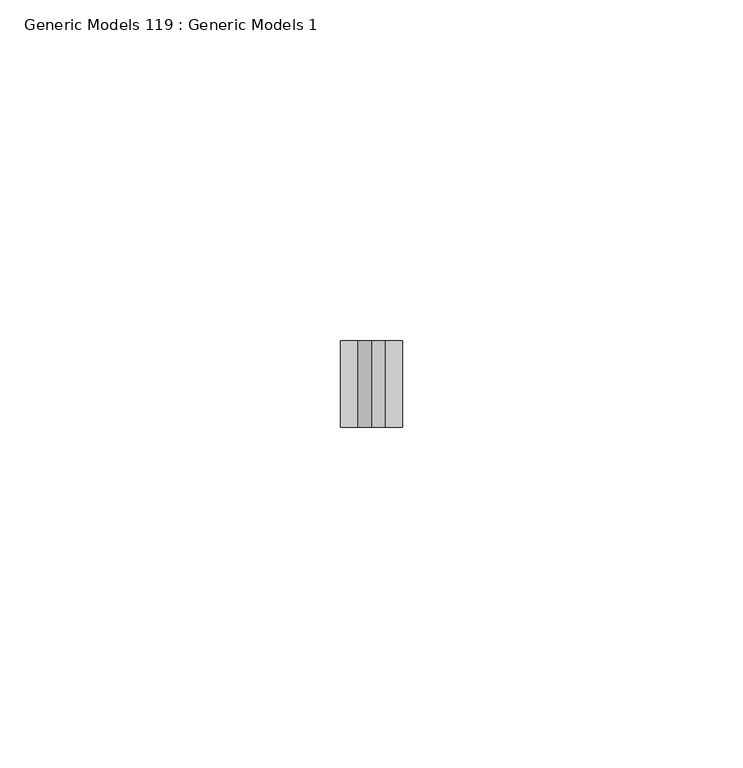
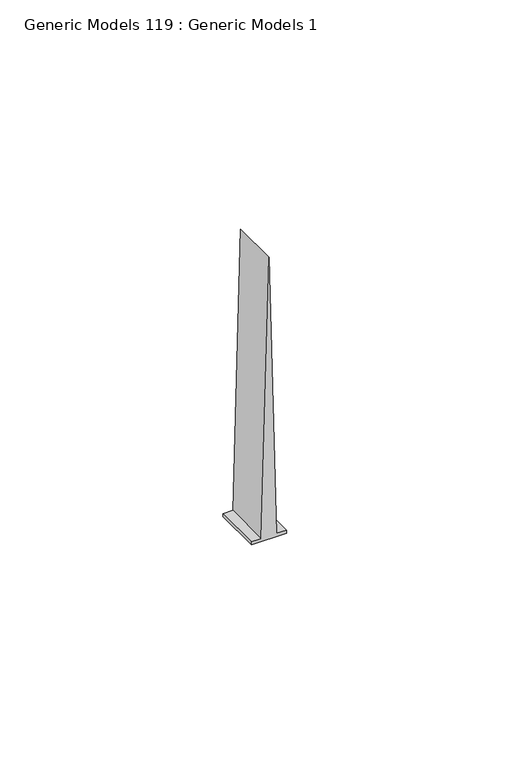
"""IFC4 building model written with IfcOpenShell, lengths in millimetres: proxy geometry, Generic Models 119 : Generic Models 1."""

from ifc_helpers import new_model, si_unit, frame, origin, place, context, project, spatial, polyline, outline, extrude, source, transform, mapped, element, save


def generic_models_119_generic_models_1_00b115a0(model_context):
    return source(origin(), model_context, "Body", "SweptSolid", [
        extrude(outline(polyline([(2429.7615469, 49845.474547), (2429.7615469, 49854.567747), (2430.5552969, 49854.567747), (2430.5552969, 49852.0178834), (2506.7552969, 49850.021147), (2430.5552969, 49848.0244106), (2430.5552969, 49845.474547), (2429.7615469, 49845.474547)])), frame((0.0, 565.15, 0.0), z_axis=(0.0, 1.0, 0.0), x_axis=(0.0, 0.0, 1.0)), (0.0, 0.0, 1.0), 12.7),
    ])


if __name__ == "__main__":
    model = new_model("IFC4")
    model_context = context("Model", 3, world=origin())
    ifc_project = project(units=[si_unit("LENGTHUNIT", "METRE", prefix="MILLI")], contexts=[model_context])
    site = spatial("IfcSite", under=ifc_project)
    building = spatial("IfcBuilding", under=site)
    placement = place(None, origin())
    generic_models_119_generic_models_1_shape = generic_models_119_generic_models_1_00b115a0(model_context)
    element("IfcBuildingElementProxy", 1, Name="Generic Models 119 : Generic Models 1", ObjectType="Generic Models 119 : Generic Models 1", at=placement, inside=building, context=model_context, shape_type="MappedRepresentation", body=[
        mapped(generic_models_119_generic_models_1_shape, transform((0.0, 0.0, 0.0), x_axis=(1.0, 0.0, 0.0), y_axis=(0.0, 1.0, 0.0), z_axis=(0.0, 0.0, 1.0))),
    ])
    save(model, "model.ifc")

# Revit data of these elements
# Element 1 (IfcBuildingElementProxy, "Generic Models 119 : Generic Models 1")
#   Materials on its faces: "ATTACH GYPSUM BOARD TO STUDS AND NOT TO TOP TRACK"
# Materials
#   "ATTACH GYPSUM BOARD TO STUDS AND NOT TO TOP TRACK": class "Generic", colour RGB 48 48 48, transparency 0, Cost = 0
